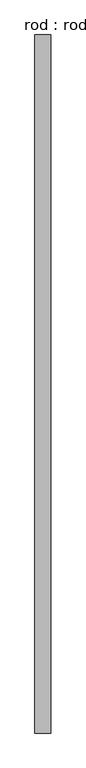
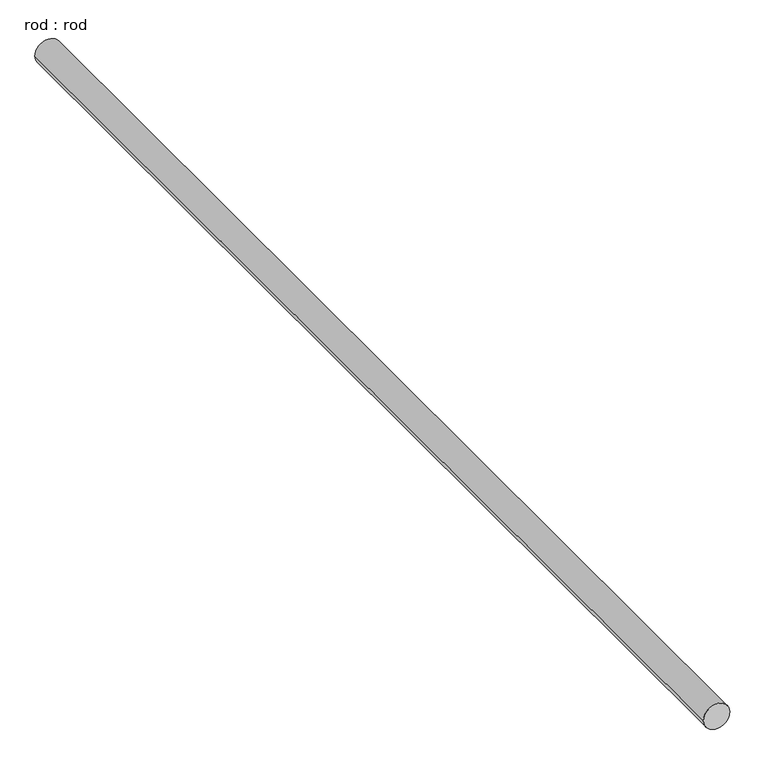
"""IFC4 building model written with IfcOpenShell, lengths in millimetres: proxy geometry, rod : rod."""

import ifcopenshell
import ifcopenshell.guid

model = None  # the IFC model being written
_history = None  # IfcOwnerHistory: only IFC2X3 demands one
_inside = {}  # id of a spatial element -> (the spatial element, [elements in it])
_under = {}  # id of a project, library or spatial element -> (it, [spatial elements below it])
_declared = {}  # id of a project -> (the project, [libraries it declares])
_typed = {}  # id of a type object -> (the type object, [elements of that type])
_made_of = {}  # id of a material, layer set ... -> (it, [elements and type objects made of it])


def new_model(schema):
    """Start an empty IFC model of exactly this schema.

    Asked for "IFC4X3", IfcOpenShell would pick the latest addendum, in which some entities
    have other attributes; the version numbers below select the first issue.
    IFC2X3 requires an IfcOwnerHistory on every rooted entity: one is made here for all.
    """
    global model, _history
    if schema == "IFC4X3":
        model = ifcopenshell.file(schema_version=(4, 3, 0, 0))
    else:
        model = ifcopenshell.file(schema=schema)
    _inside.clear()
    _under.clear()
    _declared.clear()
    _typed.clear()
    _made_of.clear()
    _history = None
    if model.schema == "IFC2X3":
        org = make("IfcOrganization", Name="unknown")
        user = make(
            "IfcPersonAndOrganization",
            ThePerson=make("IfcPerson", FamilyName="unknown"),
            TheOrganization=org,
        )
        app = make(
            "IfcApplication",
            ApplicationDeveloper=org,
            Version="unknown",
            ApplicationFullName="unknown",
            ApplicationIdentifier="unknown",
        )
        _history = make(
            "IfcOwnerHistory",
            OwningUser=user,
            OwningApplication=app,
            ChangeAction="ADDED",
            CreationDate=0,
        )
    return model


def make(cls, **values):
    """One entity of the class cls with the attributes given. An attribute that is None is left unset."""
    return model.create_entity(
        cls, **{name: value for name, value in values.items() if value is not None}
    )


def rooted(cls, **values):
    """An entity with a GlobalId (a new one), such as an element, a storey or a relation."""
    return make(cls, GlobalId=ifcopenshell.guid.new(), OwnerHistory=_history, **values)


def si_unit(unit_type, name, prefix=None):
    """IfcSIUnit, for example si_unit("LENGTHUNIT", "METRE", prefix="MILLI")."""
    return make("IfcSIUnit", UnitType=unit_type, Prefix=prefix, Name=name)


def assignment(units):
    """IfcUnitAssignment: the units of a project."""
    return None if units is None else make("IfcUnitAssignment", Units=units)


def point(xyz):
    """IfcCartesianPoint."""
    return None if xyz is None else make("IfcCartesianPoint", Coordinates=xyz)


def direction(xyz):
    """IfcDirection."""
    return None if xyz is None else make("IfcDirection", DirectionRatios=xyz)


def frame(location, z_axis=None, x_axis=None):
    """IfcAxis2Placement3D, a coordinate frame: its origin and axes. An axis left out is left unset."""
    return make(
        "IfcAxis2Placement3D",
        Location=point(location),
        Axis=direction(z_axis),
        RefDirection=direction(x_axis),
    )


def frame_2d(location, x_axis=None):
    """IfcAxis2Placement2D, a coordinate frame in the plane: its origin and x axis."""
    return make(
        "IfcAxis2Placement2D", Location=point(location), RefDirection=direction(x_axis)
    )


def origin():
    """The frame at (0, 0, 0) with its axes left unset."""
    return frame((0.0, 0.0, 0.0))


def place(relative_to, where):
    """IfcLocalPlacement: puts the frame where relative to a parent placement (None: the world)."""
    return make(
        "IfcLocalPlacement", PlacementRelTo=relative_to, RelativePlacement=where
    )


def context(
    kind, dimensions, precision=None, world=None, true_north=None, identifier=None
):
    """IfcGeometricRepresentationContext, for example the 3D "Model" context."""
    return make(
        "IfcGeometricRepresentationContext",
        ContextIdentifier=identifier,
        ContextType=kind,
        CoordinateSpaceDimension=dimensions,
        Precision=precision,
        WorldCoordinateSystem=world,
        TrueNorth=true_north,
    )


def project(units=None, contexts=None):
    """IfcProject with its units and contexts."""
    return rooted(
        "IfcProject",
        Name="project",
        RepresentationContexts=contexts,
        UnitsInContext=assignment(units),
    )


def spatial(cls, under=None, at=None, **own):
    """A site, building, storey or space (cls), placed at a placement, below another one or the project."""
    s = rooted(cls, ObjectPlacement=at, **own)
    if under is not None:
        _under.setdefault(under.id(), (under, []))[1].append(s)
    return s


def circle_curve(where, radius):
    """IfcCircle in the frame where."""
    return make("IfcCircle", Position=where, Radius=radius)


def trimmed(basis, trim1, trim2, sense, master):
    """IfcTrimmedCurve: the piece of a basis curve between two trims."""
    return make(
        "IfcTrimmedCurve",
        BasisCurve=basis,
        Trim1=trim1,
        Trim2=trim2,
        SenseAgreement=sense,
        MasterRepresentation=master,
    )


def segment(curve, same_sense, transition):
    """IfcCompositeCurveSegment."""
    return make(
        "IfcCompositeCurveSegment",
        Transition=transition,
        SameSense=same_sense,
        ParentCurve=curve,
    )


def composite_curve(segments, self_intersect=None):
    """IfcCompositeCurve: segments joined end to end."""
    return make("IfcCompositeCurve", Segments=segments, SelfIntersect=self_intersect)


def outline(outer, holes=None, kind="AREA"):
    """IfcArbitraryClosedProfileDef: a profile drawn as a closed curve; with holes, ...WithVoids."""
    if holes is None:
        return make("IfcArbitraryClosedProfileDef", ProfileType=kind, OuterCurve=outer)
    return make(
        "IfcArbitraryProfileDefWithVoids",
        ProfileType=kind,
        OuterCurve=outer,
        InnerCurves=holes,
    )


def extrude(swept, where, along, depth):
    """IfcExtrudedAreaSolid: the profile swept, set in the frame where, extruded along a direction by depth."""
    return make(
        "IfcExtrudedAreaSolid",
        SweptArea=swept,
        Position=where,
        ExtrudedDirection=direction(along),
        Depth=depth,
    )


def shape(context_of_items, identifier, shape_type, items):
    """IfcShapeRepresentation: the items that make up one representation, for example the "Body"."""
    return make(
        "IfcShapeRepresentation",
        ContextOfItems=context_of_items,
        RepresentationIdentifier=identifier,
        RepresentationType=shape_type,
        Items=items,
    )


def source(mapping_origin, context_of_items, identifier, shape_type, items):
    """IfcRepresentationMap: a shape defined once, which mapped items show again and again."""
    return make(
        "IfcRepresentationMap",
        MappingOrigin=mapping_origin,
        MappedRepresentation=shape(context_of_items, identifier, shape_type, items),
    )


def transform(
    local_origin,
    x_axis=None,
    y_axis=None,
    z_axis=None,
    scale=None,
    scale2=None,
    scale3=None,
    uniform=True,
):
    """IfcCartesianTransformationOperator3D, or its non-uniform kind. x_axis, y_axis, z_axis: its Axis1, 2, 3."""
    if uniform:
        return make(
            "IfcCartesianTransformationOperator3D",
            Axis1=direction(x_axis),
            Axis2=direction(y_axis),
            LocalOrigin=point(local_origin),
            Scale=scale,
            Axis3=direction(z_axis),
        )
    return make(
        "IfcCartesianTransformationOperator3DnonUniform",
        Axis1=direction(x_axis),
        Axis2=direction(y_axis),
        LocalOrigin=point(local_origin),
        Scale=scale,
        Axis3=direction(z_axis),
        Scale2=scale2,
        Scale3=scale3,
    )


def mapped(mapping_source, mapping_target):
    """IfcMappedItem: shows the shape of a source again, moved by a transform."""
    return make(
        "IfcMappedItem", MappingSource=mapping_source, MappingTarget=mapping_target
    )


def made_of(thing, what):
    """Note that an element or type object is made of a material, layer set ...; save() writes the relation."""
    if what is not None:
        _made_of.setdefault(what.id(), (what, []))[1].append(thing)
    return thing


def element(
    cls,
    number,
    at=None,
    inside=None,
    cuts=None,
    type_object=None,
    material=None,
    context=None,
    identifier="Body",
    shape_type=None,
    held_by="IfcProductDefinitionShape",
    body=None,
    shapes=None,
    **own,
):
    """One element of the class cls, such as IfcWall. Its Tag is "e" and its number.

    at: its placement. inside: the storey or other place that contains it. cuts: it is an
    opening in that element (IfcRelVoidsElement). A single representation is given by context,
    identifier, shape_type and body (its items); several are given by shapes. held_by: the class
    of the entity that holds the representations. save() writes the other relations.
    """
    e = rooted(cls, Tag="e%d" % number, ObjectPlacement=at, **own)
    if body is not None:
        shapes = [shape(context, identifier, shape_type, body)]
    if shapes is not None:
        e.Representation = make(held_by, Representations=shapes)
    if inside is not None:
        _inside.setdefault(inside.id(), (inside, []))[1].append(e)
    if cuts is not None:
        rooted(
            "IfcRelVoidsElement", RelatingBuildingElement=cuts, RelatedOpeningElement=e
        )
    if type_object is not None:
        _typed.setdefault(type_object.id(), (type_object, []))[1].append(e)
    return made_of(e, material)


def aggregate(whole, parts):
    """IfcRelAggregates: a whole, such as a stair, and the parts it consists of."""
    return rooted("IfcRelAggregates", RelatingObject=whole, RelatedObjects=parts)


def save(model, path):
    """Write the relations noted so far, then the file.

    IfcRelAggregates (storeys below a building ...), IfcRelContainedInSpatialStructure (elements
    in a storey), IfcRelDefinesByType, IfcRelAssociatesMaterial and IfcRelDeclares: one each for
    every whole, place, type object, material and project.
    """
    for whole, parts in _under.values():
        aggregate(whole, parts)
    for where, things in _inside.values():
        rooted(
            "IfcRelContainedInSpatialStructure",
            RelatedElements=things,
            RelatingStructure=where,
        )
    for kind, things in _typed.values():
        rooted("IfcRelDefinesByType", RelatedObjects=things, RelatingType=kind)
    for what, things in _made_of.values():
        rooted("IfcRelAssociatesMaterial", RelatedObjects=things, RelatingMaterial=what)
    for by, libraries in _declared.values():
        rooted("IfcRelDeclares", RelatingContext=by, RelatedDefinitions=libraries)
    model.write(path)


def rod_rod_e6bf28ec(model_context):
    return source(origin(), model_context, "Body", "SweptSolid", [
        extrude(outline(composite_curve([segment(trimmed(circle_curve(frame_2d((0.0108462, 0.0)), 200.0), [point((0.0108462, 200.0))], [point((0.0108462, -200.0))], False, "CARTESIAN"), True, "CONTINUOUS"), segment(trimmed(circle_curve(frame_2d((0.0108462, 0.0)), 200.0), [point((0.0108462, -200.0))], [point((0.0108462, 200.0))], False, "CARTESIAN"), True, "CONTINUOUS")], self_intersect=False)), frame((0.0, -4714.2400207, 0.0), z_axis=(0.0, 1.0, 0.0), x_axis=(0.0, 0.0, 1.0)), (0.0, 0.0, 1.0), 17613.9372721),
    ])


if __name__ == "__main__":
    model = new_model("IFC4")
    model_context = context("Model", 3, world=origin())
    ifc_project = project(units=[si_unit("LENGTHUNIT", "METRE", prefix="MILLI")], contexts=[model_context])
    site = spatial("IfcSite", under=ifc_project)
    building = spatial("IfcBuilding", under=site)
    placement = place(None, origin())
    rod_rod_shape = rod_rod_e6bf28ec(model_context)
    element("IfcBuildingElementProxy", 1, Name="rod : rod", ObjectType="rod : rod", at=placement, inside=building, context=model_context, shape_type="MappedRepresentation", body=[
        mapped(rod_rod_shape, transform((0.0, 0.0, 0.0), x_axis=(1.0, 0.0, 0.0), y_axis=(0.0, 1.0, 0.0), z_axis=(0.0, 0.0, 1.0))),
    ])
    save(model, "model.ifc")

# Revit data of these elements
# Type "rod : rod"
#   Default Elevation = 0
